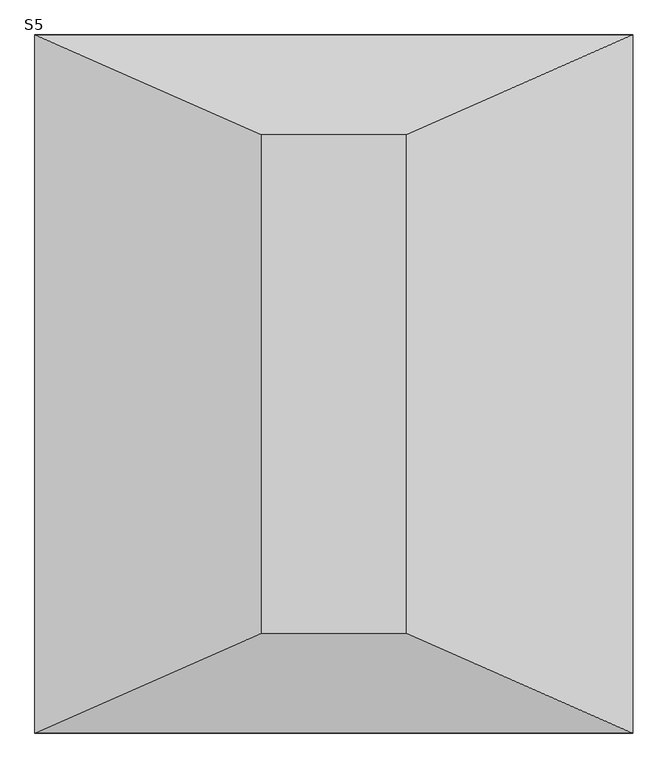
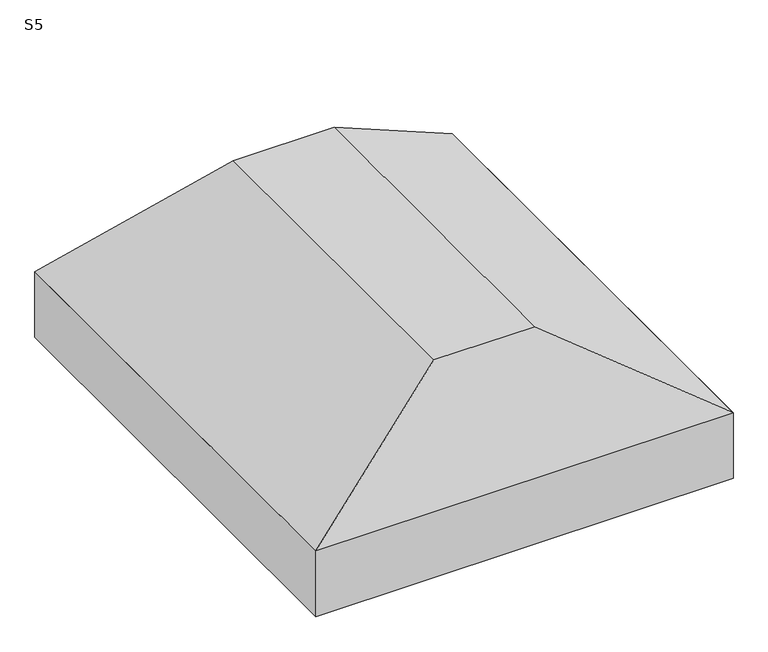
"""IFC4 building model written with IfcOpenShell, lengths in millimetres: fastener geometry, TQS - Sapata : S5."""

from ifc_helpers import new_model, si_unit, frame, origin, place, context, project, spatial, polyline, outline, extrude, faceted_brep, source, transform, mapped, element, save


def s5_cab1d6eb(model_context):
    return source(origin(), model_context, "Body", "SolidModel", [
        faceted_brep([(-55.0, 300.0, 0.0), (-345.0, 300.0, 0.0), (-345.0, -700.0, 0.0), (-55.0, -700.0, 0.0), (400.0, 500.0, -300.0), (400.0, -900.0, -300.0), (-800.0, -900.0, -300.0), (-800.0, 500.0, -300.0)], [[[0, 1, 2, 3]], [[4, 5, 6, 7]], [[4, 7, 1, 0]], [[7, 6, 2, 1]], [[6, 5, 3, 2]], [[5, 4, 0, 3]]]),
        extrude(outline(polyline([(400.0, 500.0), (400.0, -900.0), (-800.0, -900.0), (-800.0, 500.0), (400.0, 500.0)])), frame((0.0, 0.0, -500.0), z_axis=(0.0, 0.0, 1.0), x_axis=(1.0, 0.0, 0.0)), (0.0, 0.0, 1.0), 200.0),
    ])


if __name__ == "__main__":
    model = new_model("IFC4")
    model_context = context("Model", 3, world=origin())
    ifc_project = project(units=[si_unit("LENGTHUNIT", "METRE", prefix="MILLI")], contexts=[model_context])
    site = spatial("IfcSite", under=ifc_project)
    building = spatial("IfcBuilding", under=site)
    placement = place(None, origin())
    s5_shape = s5_cab1d6eb(model_context)
    element("IfcFastener", 1, ObjectType="TQS - Sapata : S5", at=placement, inside=building, context=model_context, shape_type="MappedRepresentation", body=[
        mapped(s5_shape, transform((0.0, 0.0, 0.0), x_axis=(1.0, 0.0, 0.0), y_axis=(0.0, 1.0, 0.0), z_axis=(0.0, 0.0, 1.0))),
    ])
    save(model, "model.ifc")

# Revit data of these elements
# Type "TQS - Sapata : S5"
#   TY = 1.00 m
#   TX = 0.29 m
#   HS = 0.50 m
#   H0 = 0.20 m
#   EXCYABS = 0.70 m
#   EXCY = 0.00 m
#   EXCXABS = 0.60 m
#   EXCX = 0.00 m
#   DIMY = 1.40 m
#   DIMX = 1.20 m
#   Material estrutural = Concreto - Concreto concretado no local
#   Width = 0
#   Length = 0
# Element 1 (IfcFastener, "TQS - Sapata : S5")
#   Materials on its faces: "Concreto - Concreto concretado no local"
# Materials
#   "Concreto - Concreto concretado no local": class "Concreto", colour RGB 192 192 192, transparency 0
